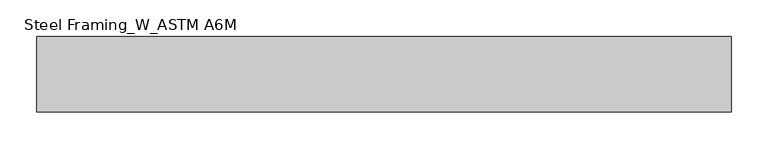
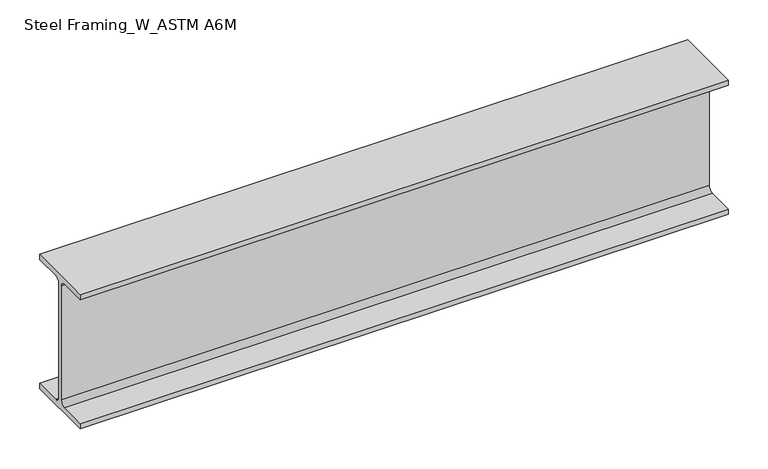
"""IFC4 building model written with IfcOpenShell, lengths in millimetres: beam geometry, Steel Framing_W_ASTM A6M : H_SB_AR_S02_W200x22.5_J1."""

import ifcopenshell
import ifcopenshell.guid

model = None  # the IFC model being written
_history = None  # IfcOwnerHistory: only IFC2X3 demands one
_inside = {}  # id of a spatial element -> (the spatial element, [elements in it])
_under = {}  # id of a project, library or spatial element -> (it, [spatial elements below it])
_declared = {}  # id of a project -> (the project, [libraries it declares])
_typed = {}  # id of a type object -> (the type object, [elements of that type])
_made_of = {}  # id of a material, layer set ... -> (it, [elements and type objects made of it])


def new_model(schema):
    """Start an empty IFC model of exactly this schema.

    Asked for "IFC4X3", IfcOpenShell would pick the latest addendum, in which some entities
    have other attributes; the version numbers below select the first issue.
    IFC2X3 requires an IfcOwnerHistory on every rooted entity: one is made here for all.
    """
    global model, _history
    if schema == "IFC4X3":
        model = ifcopenshell.file(schema_version=(4, 3, 0, 0))
    else:
        model = ifcopenshell.file(schema=schema)
    _inside.clear()
    _under.clear()
    _declared.clear()
    _typed.clear()
    _made_of.clear()
    _history = None
    if model.schema == "IFC2X3":
        org = make("IfcOrganization", Name="unknown")
        user = make(
            "IfcPersonAndOrganization",
            ThePerson=make("IfcPerson", FamilyName="unknown"),
            TheOrganization=org,
        )
        app = make(
            "IfcApplication",
            ApplicationDeveloper=org,
            Version="unknown",
            ApplicationFullName="unknown",
            ApplicationIdentifier="unknown",
        )
        _history = make(
            "IfcOwnerHistory",
            OwningUser=user,
            OwningApplication=app,
            ChangeAction="ADDED",
            CreationDate=0,
        )
    return model


def make(cls, **values):
    """One entity of the class cls with the attributes given. An attribute that is None is left unset."""
    return model.create_entity(
        cls, **{name: value for name, value in values.items() if value is not None}
    )


def rooted(cls, **values):
    """An entity with a GlobalId (a new one), such as an element, a storey or a relation."""
    return make(cls, GlobalId=ifcopenshell.guid.new(), OwnerHistory=_history, **values)


def si_unit(unit_type, name, prefix=None):
    """IfcSIUnit, for example si_unit("LENGTHUNIT", "METRE", prefix="MILLI")."""
    return make("IfcSIUnit", UnitType=unit_type, Prefix=prefix, Name=name)


def assignment(units):
    """IfcUnitAssignment: the units of a project."""
    return None if units is None else make("IfcUnitAssignment", Units=units)


def point(xyz):
    """IfcCartesianPoint."""
    return None if xyz is None else make("IfcCartesianPoint", Coordinates=xyz)


def direction(xyz):
    """IfcDirection."""
    return None if xyz is None else make("IfcDirection", DirectionRatios=xyz)


def frame(location, z_axis=None, x_axis=None):
    """IfcAxis2Placement3D, a coordinate frame: its origin and axes. An axis left out is left unset."""
    return make(
        "IfcAxis2Placement3D",
        Location=point(location),
        Axis=direction(z_axis),
        RefDirection=direction(x_axis),
    )


def frame_2d(location, x_axis=None):
    """IfcAxis2Placement2D, a coordinate frame in the plane: its origin and x axis."""
    return make(
        "IfcAxis2Placement2D", Location=point(location), RefDirection=direction(x_axis)
    )


def origin():
    """The frame at (0, 0, 0) with its axes left unset."""
    return frame((0.0, 0.0, 0.0))


def place(relative_to, where):
    """IfcLocalPlacement: puts the frame where relative to a parent placement (None: the world)."""
    return make(
        "IfcLocalPlacement", PlacementRelTo=relative_to, RelativePlacement=where
    )


def context(
    kind, dimensions, precision=None, world=None, true_north=None, identifier=None
):
    """IfcGeometricRepresentationContext, for example the 3D "Model" context."""
    return make(
        "IfcGeometricRepresentationContext",
        ContextIdentifier=identifier,
        ContextType=kind,
        CoordinateSpaceDimension=dimensions,
        Precision=precision,
        WorldCoordinateSystem=world,
        TrueNorth=true_north,
    )


def project(units=None, contexts=None):
    """IfcProject with its units and contexts."""
    return rooted(
        "IfcProject",
        Name="project",
        RepresentationContexts=contexts,
        UnitsInContext=assignment(units),
    )


def spatial(cls, under=None, at=None, **own):
    """A site, building, storey or space (cls), placed at a placement, below another one or the project."""
    s = rooted(cls, ObjectPlacement=at, **own)
    if under is not None:
        _under.setdefault(under.id(), (under, []))[1].append(s)
    return s


def polyline(points):
    """IfcPolyline through the points."""
    return make("IfcPolyline", Points=[point(p) for p in points])


def circle_curve(where, radius):
    """IfcCircle in the frame where."""
    return make("IfcCircle", Position=where, Radius=radius)


def trimmed(basis, trim1, trim2, sense, master):
    """IfcTrimmedCurve: the piece of a basis curve between two trims."""
    return make(
        "IfcTrimmedCurve",
        BasisCurve=basis,
        Trim1=trim1,
        Trim2=trim2,
        SenseAgreement=sense,
        MasterRepresentation=master,
    )


def segment(curve, same_sense, transition):
    """IfcCompositeCurveSegment."""
    return make(
        "IfcCompositeCurveSegment",
        Transition=transition,
        SameSense=same_sense,
        ParentCurve=curve,
    )


def composite_curve(segments, self_intersect=None):
    """IfcCompositeCurve: segments joined end to end."""
    return make("IfcCompositeCurve", Segments=segments, SelfIntersect=self_intersect)


def outline(outer, holes=None, kind="AREA"):
    """IfcArbitraryClosedProfileDef: a profile drawn as a closed curve; with holes, ...WithVoids."""
    if holes is None:
        return make("IfcArbitraryClosedProfileDef", ProfileType=kind, OuterCurve=outer)
    return make(
        "IfcArbitraryProfileDefWithVoids",
        ProfileType=kind,
        OuterCurve=outer,
        InnerCurves=holes,
    )


def extrude(swept, where, along, depth):
    """IfcExtrudedAreaSolid: the profile swept, set in the frame where, extruded along a direction by depth."""
    return make(
        "IfcExtrudedAreaSolid",
        SweptArea=swept,
        Position=where,
        ExtrudedDirection=direction(along),
        Depth=depth,
    )


def shape(context_of_items, identifier, shape_type, items):
    """IfcShapeRepresentation: the items that make up one representation, for example the "Body"."""
    return make(
        "IfcShapeRepresentation",
        ContextOfItems=context_of_items,
        RepresentationIdentifier=identifier,
        RepresentationType=shape_type,
        Items=items,
    )


def source(mapping_origin, context_of_items, identifier, shape_type, items):
    """IfcRepresentationMap: a shape defined once, which mapped items show again and again."""
    return make(
        "IfcRepresentationMap",
        MappingOrigin=mapping_origin,
        MappedRepresentation=shape(context_of_items, identifier, shape_type, items),
    )


def transform(
    local_origin,
    x_axis=None,
    y_axis=None,
    z_axis=None,
    scale=None,
    scale2=None,
    scale3=None,
    uniform=True,
):
    """IfcCartesianTransformationOperator3D, or its non-uniform kind. x_axis, y_axis, z_axis: its Axis1, 2, 3."""
    if uniform:
        return make(
            "IfcCartesianTransformationOperator3D",
            Axis1=direction(x_axis),
            Axis2=direction(y_axis),
            LocalOrigin=point(local_origin),
            Scale=scale,
            Axis3=direction(z_axis),
        )
    return make(
        "IfcCartesianTransformationOperator3DnonUniform",
        Axis1=direction(x_axis),
        Axis2=direction(y_axis),
        LocalOrigin=point(local_origin),
        Scale=scale,
        Axis3=direction(z_axis),
        Scale2=scale2,
        Scale3=scale3,
    )


def mapped(mapping_source, mapping_target):
    """IfcMappedItem: shows the shape of a source again, moved by a transform."""
    return make(
        "IfcMappedItem", MappingSource=mapping_source, MappingTarget=mapping_target
    )


def made_of(thing, what):
    """Note that an element or type object is made of a material, layer set ...; save() writes the relation."""
    if what is not None:
        _made_of.setdefault(what.id(), (what, []))[1].append(thing)
    return thing


def element(
    cls,
    number,
    at=None,
    inside=None,
    cuts=None,
    type_object=None,
    material=None,
    context=None,
    identifier="Body",
    shape_type=None,
    held_by="IfcProductDefinitionShape",
    body=None,
    shapes=None,
    **own,
):
    """One element of the class cls, such as IfcWall. Its Tag is "e" and its number.

    at: its placement. inside: the storey or other place that contains it. cuts: it is an
    opening in that element (IfcRelVoidsElement). A single representation is given by context,
    identifier, shape_type and body (its items); several are given by shapes. held_by: the class
    of the entity that holds the representations. save() writes the other relations.
    """
    e = rooted(cls, Tag="e%d" % number, ObjectPlacement=at, **own)
    if body is not None:
        shapes = [shape(context, identifier, shape_type, body)]
    if shapes is not None:
        e.Representation = make(held_by, Representations=shapes)
    if inside is not None:
        _inside.setdefault(inside.id(), (inside, []))[1].append(e)
    if cuts is not None:
        rooted(
            "IfcRelVoidsElement", RelatingBuildingElement=cuts, RelatedOpeningElement=e
        )
    if type_object is not None:
        _typed.setdefault(type_object.id(), (type_object, []))[1].append(e)
    return made_of(e, material)


def aggregate(whole, parts):
    """IfcRelAggregates: a whole, such as a stair, and the parts it consists of."""
    return rooted("IfcRelAggregates", RelatingObject=whole, RelatedObjects=parts)


def save(model, path):
    """Write the relations noted so far, then the file.

    IfcRelAggregates (storeys below a building ...), IfcRelContainedInSpatialStructure (elements
    in a storey), IfcRelDefinesByType, IfcRelAssociatesMaterial and IfcRelDeclares: one each for
    every whole, place, type object, material and project.
    """
    for whole, parts in _under.values():
        aggregate(whole, parts)
    for where, things in _inside.values():
        rooted(
            "IfcRelContainedInSpatialStructure",
            RelatedElements=things,
            RelatingStructure=where,
        )
    for kind, things in _typed.values():
        rooted("IfcRelDefinesByType", RelatedObjects=things, RelatingType=kind)
    for what, things in _made_of.values():
        rooted("IfcRelAssociatesMaterial", RelatedObjects=things, RelatingMaterial=what)
    for by, libraries in _declared.values():
        rooted("IfcRelDeclares", RelatingContext=by, RelatedDefinitions=libraries)
    model.write(path)


def steel_framing_w_astm_a6m_f3cc38eb(model_context):
    return source(origin(), model_context, "Body", "SweptSolid", [
        extrude(outline(composite_curve([segment(polyline([(51.0, -95.0), (51.0, -103.0), (-51.0, -103.0), (-51.0, -95.0), (-10.71, -95.0)]), True, "CONTINUOUS"), segment(trimmed(circle_curve(frame_2d((-10.71, -87.4)), 7.6), [point((-10.71, -95.0))], [point((-3.11, -87.4))], True, "CARTESIAN"), True, "CONTINUOUS"), segment(polyline([(-3.11, -87.4), (-3.11, 87.4)]), True, "CONTINUOUS"), segment(trimmed(circle_curve(frame_2d((-10.71, 87.4)), 7.6), [point((-3.11, 87.4))], [point((-10.71, 95.0))], True, "CARTESIAN"), True, "CONTINUOUS"), segment(polyline([(-10.71, 95.0), (-51.0, 95.0), (-51.0, 103.0), (51.0, 103.0), (51.0, 95.0), (10.71, 95.0)]), True, "CONTINUOUS"), segment(trimmed(circle_curve(frame_2d((10.71, 87.4)), 7.6), [point((10.71, 95.0))], [point((3.11, 87.4))], True, "CARTESIAN"), True, "CONTINUOUS"), segment(polyline([(3.11, 87.4), (3.11, -87.4)]), True, "CONTINUOUS"), segment(trimmed(circle_curve(frame_2d((10.71, -87.4)), 7.6), [point((3.11, -87.4))], [point((10.71, -95.0))], True, "CARTESIAN"), True, "CONTINUOUS"), segment(polyline([(10.71, -95.0), (51.0, -95.0)]), True, "CONTINUOUS")], self_intersect=False)), frame((-470.3, 0.0, 0.0), z_axis=(1.0, 0.0, 0.0), x_axis=(0.0, 1.0, 0.0)), (0.0, 0.0, 1.0), 940.6),
    ])


if __name__ == "__main__":
    model = new_model("IFC4")
    model_context = context("Model", 3, world=origin())
    ifc_project = project(units=[si_unit("LENGTHUNIT", "METRE", prefix="MILLI")], contexts=[model_context])
    site = spatial("IfcSite", under=ifc_project)
    building = spatial("IfcBuilding", under=site)
    placement = place(None, origin())
    steel_framing_w_astm_a6m_shape = steel_framing_w_astm_a6m_f3cc38eb(model_context)
    element("IfcBeam", 1, ObjectType="Steel Framing_W_ASTM A6M : H_SB_AR_S02_W200x22.5_J1", at=placement, inside=building, context=model_context, shape_type="MappedRepresentation", body=[
        mapped(steel_framing_w_astm_a6m_shape, transform((0.0, 0.0, 0.0), x_axis=(1.0, 0.0, 0.0), y_axis=(0.0, 1.0, 0.0), z_axis=(0.0, 0.0, 1.0))),
    ])
    save(model, "model.ifc")

# Revit data of these elements
# Type "Steel Framing_W_ASTM A6M : H_SB_AR_S02_W200x22.5_J1"
#   Section Name Key = "W8x15"
#   Width = 10.2 cm
#   Web Thickness = 0.622 cm
#   Web Fillet = 0.76 cm
#   Warping Constant = 13900.0 cm⁶
#   Torsional Moment of Inertia = 5.70 cm⁴
#   Section Area = 28.6 cm²
#   Plastic Modulus weak axis = 43.8 cm³
#   Plastic Modulus strong axis = 223.0 cm³
#   Perimeter = 0.795 m²/m
#   Nominal Weight = 22.50 kgf/m
#   Moment of Inertia weak axis = 142.00 cm⁴
#   Moment of Inertia strong axis = 2000.00 cm⁴
#   Height = 20.6 cm
#   Flange Thickness = 0.8 cm
#   Elastic Modulus weak axis = 27.9 cm³
#   Elastic Modulus strong axis = 193.0 cm³
#   Centroid Vertical = 10.3 cm
#   Centroid Horizontal = 5.1 cm
#   Length [instance default] = 1500 mm
#   Structural Material [instance default] = Steel, 45-345
#   Bolt Spacing = 0
#   Assembly Code = ""
# Element 1 (IfcBeam, "Steel Framing_W_ASTM A6M : H_SB_AR_S02_W200x22.5_J1")
#   Materials on its faces: "Steel, 45-345"
# Materials
#   "Steel, 45-345": class "Metal", colour RGB 189 187 185, transparency 0, Description = "Steel 345 MPa", Cost = 0
